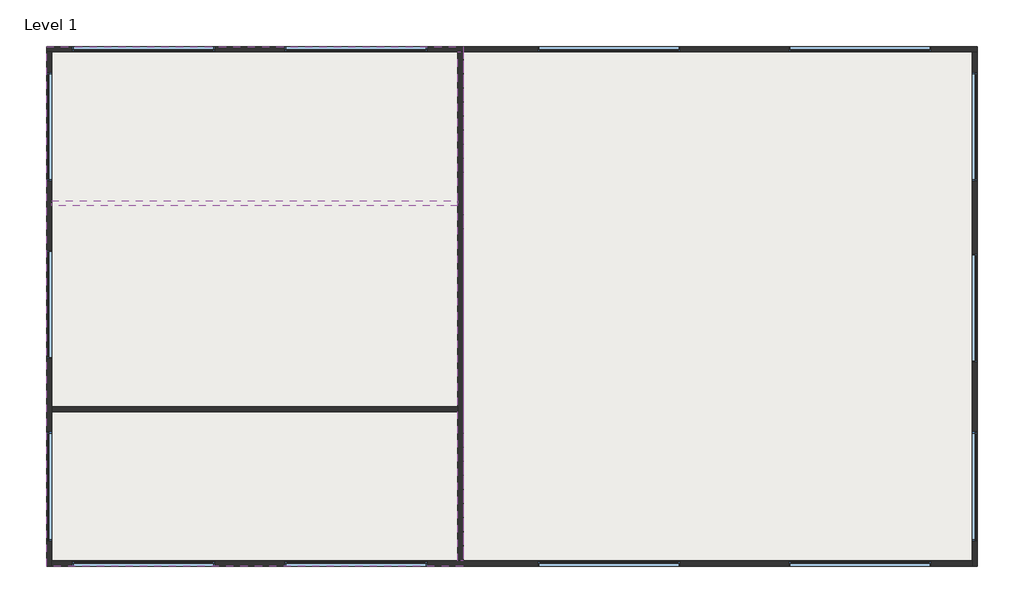
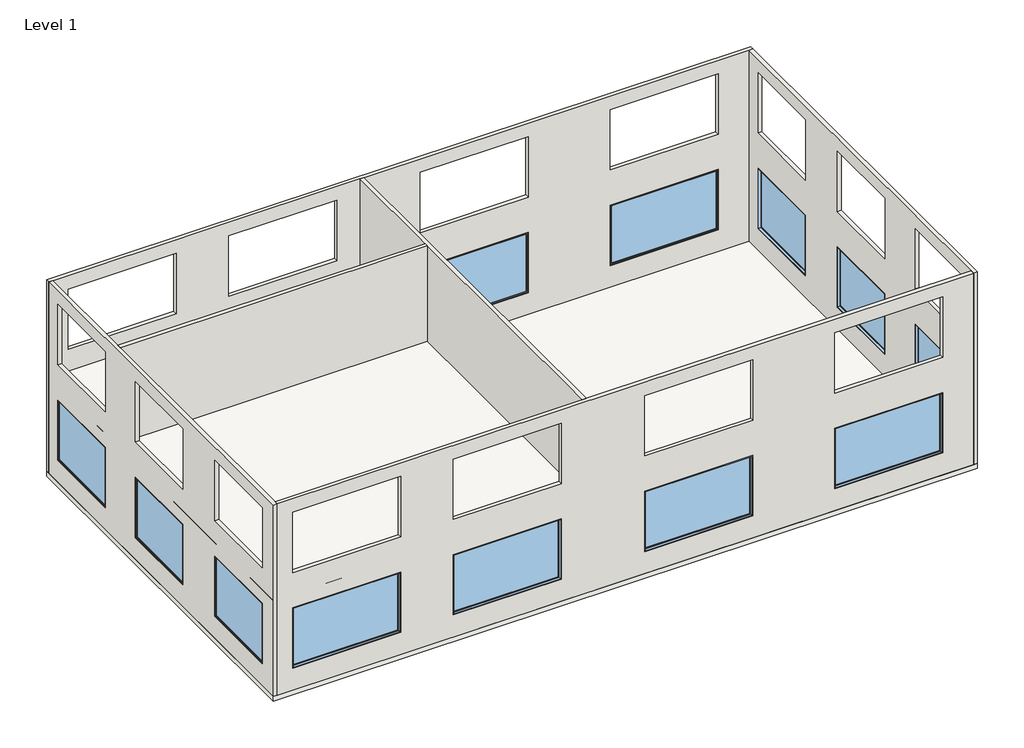
# One storey: 14 windows, 8 walls, 2 slabs.
"""IFC4 building model written with IfcOpenShell, lengths in millimetres."""

import ifcopenshell
import ifcopenshell.guid

model = None  # the IFC model being written
_history = None  # IfcOwnerHistory: only IFC2X3 demands one
_inside = {}  # id of a spatial element -> (the spatial element, [elements in it])
_under = {}  # id of a project, library or spatial element -> (it, [spatial elements below it])
_declared = {}  # id of a project -> (the project, [libraries it declares])
_typed = {}  # id of a type object -> (the type object, [elements of that type])
_made_of = {}  # id of a material, layer set ... -> (it, [elements and type objects made of it])


def new_model(schema):
    """Start an empty IFC model of exactly this schema.

    Asked for "IFC4X3", IfcOpenShell would pick the latest addendum, in which some entities
    have other attributes; the version numbers below select the first issue.
    IFC2X3 requires an IfcOwnerHistory on every rooted entity: one is made here for all.
    """
    global model, _history
    if schema == "IFC4X3":
        model = ifcopenshell.file(schema_version=(4, 3, 0, 0))
    else:
        model = ifcopenshell.file(schema=schema)
    _inside.clear()
    _under.clear()
    _declared.clear()
    _typed.clear()
    _made_of.clear()
    _history = None
    if model.schema == "IFC2X3":
        org = make("IfcOrganization", Name="unknown")
        user = make(
            "IfcPersonAndOrganization",
            ThePerson=make("IfcPerson", FamilyName="unknown"),
            TheOrganization=org,
        )
        app = make(
            "IfcApplication",
            ApplicationDeveloper=org,
            Version="unknown",
            ApplicationFullName="unknown",
            ApplicationIdentifier="unknown",
        )
        _history = make(
            "IfcOwnerHistory",
            OwningUser=user,
            OwningApplication=app,
            ChangeAction="ADDED",
            CreationDate=0,
        )
    return model


def make(cls, **values):
    """One entity of the class cls with the attributes given. An attribute that is None is left unset."""
    return model.create_entity(
        cls, **{name: value for name, value in values.items() if value is not None}
    )


def rooted(cls, **values):
    """An entity with a GlobalId (a new one), such as an element, a storey or a relation."""
    return make(cls, GlobalId=ifcopenshell.guid.new(), OwnerHistory=_history, **values)


def si_unit(unit_type, name, prefix=None):
    """IfcSIUnit, for example si_unit("LENGTHUNIT", "METRE", prefix="MILLI")."""
    return make("IfcSIUnit", UnitType=unit_type, Prefix=prefix, Name=name)


def assignment(units):
    """IfcUnitAssignment: the units of a project."""
    return None if units is None else make("IfcUnitAssignment", Units=units)


def point(xyz):
    """IfcCartesianPoint."""
    return None if xyz is None else make("IfcCartesianPoint", Coordinates=xyz)


def direction(xyz):
    """IfcDirection."""
    return None if xyz is None else make("IfcDirection", DirectionRatios=xyz)


def frame(location, z_axis=None, x_axis=None):
    """IfcAxis2Placement3D, a coordinate frame: its origin and axes. An axis left out is left unset."""
    return make(
        "IfcAxis2Placement3D",
        Location=point(location),
        Axis=direction(z_axis),
        RefDirection=direction(x_axis),
    )


def origin():
    """The frame at (0, 0, 0) with its axes left unset."""
    return frame((0.0, 0.0, 0.0))


def origin_with_axes():
    """The frame at (0, 0, 0) with the z axis (0, 0, 1) and the x axis (1, 0, 0) written out."""
    return frame((0.0, 0.0, 0.0), z_axis=(0.0, 0.0, 1.0), x_axis=(1.0, 0.0, 0.0))


def place(relative_to, where):
    """IfcLocalPlacement: puts the frame where relative to a parent placement (None: the world)."""
    return make(
        "IfcLocalPlacement", PlacementRelTo=relative_to, RelativePlacement=where
    )


def context(
    kind, dimensions, precision=None, world=None, true_north=None, identifier=None
):
    """IfcGeometricRepresentationContext, for example the 3D "Model" context."""
    return make(
        "IfcGeometricRepresentationContext",
        ContextIdentifier=identifier,
        ContextType=kind,
        CoordinateSpaceDimension=dimensions,
        Precision=precision,
        WorldCoordinateSystem=world,
        TrueNorth=true_north,
    )


def project(units=None, contexts=None):
    """IfcProject with its units and contexts."""
    return rooted(
        "IfcProject",
        Name="project",
        RepresentationContexts=contexts,
        UnitsInContext=assignment(units),
    )


def spatial(cls, under=None, at=None, **own):
    """A site, building, storey or space (cls), placed at a placement, below another one or the project."""
    s = rooted(cls, ObjectPlacement=at, **own)
    if under is not None:
        _under.setdefault(under.id(), (under, []))[1].append(s)
    return s


def polyline(points):
    """IfcPolyline through the points."""
    return make("IfcPolyline", Points=[point(p) for p in points])


def outline(outer, holes=None, kind="AREA"):
    """IfcArbitraryClosedProfileDef: a profile drawn as a closed curve; with holes, ...WithVoids."""
    if holes is None:
        return make("IfcArbitraryClosedProfileDef", ProfileType=kind, OuterCurve=outer)
    return make(
        "IfcArbitraryProfileDefWithVoids",
        ProfileType=kind,
        OuterCurve=outer,
        InnerCurves=holes,
    )


def extrude(swept, where, along, depth):
    """IfcExtrudedAreaSolid: the profile swept, set in the frame where, extruded along a direction by depth."""
    return make(
        "IfcExtrudedAreaSolid",
        SweptArea=swept,
        Position=where,
        ExtrudedDirection=direction(along),
        Depth=depth,
    )


def faces_of(points, faces, orient=None, outer=None):
    """IfcFace entities. A face is a list of loops; a loop is a list of indices into points, from 0.

    orient and outer hold one flag for each loop. By default every Orientation is true, the
    first loop of a face is its IfcFaceOuterBound and the others are IfcFaceBound.
    """
    made = []
    for i, loops in enumerate(faces):
        bounds = []
        for j, loop in enumerate(loops):
            is_outer = j == 0 if outer is None else outer[i][j]
            bounds.append(
                make(
                    "IfcFaceOuterBound" if is_outer else "IfcFaceBound",
                    Bound=make("IfcPolyLoop", Polygon=[points[k] for k in loop]),
                    Orientation=True if orient is None else orient[i][j],
                )
            )
        made.append(make("IfcFace", Bounds=bounds))
    return made


def faceted_brep(points, faces, orient=None, outer=None, voids=None):
    """IfcFacetedBrep: a solid bounded by flat faces; with voids (closed shells), ...WithVoids."""
    shared = [point(p) for p in points]
    hull = make("IfcClosedShell", CfsFaces=faces_of(shared, faces, orient, outer))
    if voids is None:
        return make("IfcFacetedBrep", Outer=hull)
    return make(
        "IfcFacetedBrepWithVoids",
        Outer=hull,
        Voids=[
            make(cls, CfsFaces=faces_of(shared, fs, o, b)) for cls, fs, o, b in voids
        ],
    )


def shape(context_of_items, identifier, shape_type, items):
    """IfcShapeRepresentation: the items that make up one representation, for example the "Body"."""
    return make(
        "IfcShapeRepresentation",
        ContextOfItems=context_of_items,
        RepresentationIdentifier=identifier,
        RepresentationType=shape_type,
        Items=items,
    )


def source(mapping_origin, context_of_items, identifier, shape_type, items):
    """IfcRepresentationMap: a shape defined once, which mapped items show again and again."""
    return make(
        "IfcRepresentationMap",
        MappingOrigin=mapping_origin,
        MappedRepresentation=shape(context_of_items, identifier, shape_type, items),
    )


def transform(
    local_origin,
    x_axis=None,
    y_axis=None,
    z_axis=None,
    scale=None,
    scale2=None,
    scale3=None,
    uniform=True,
):
    """IfcCartesianTransformationOperator3D, or its non-uniform kind. x_axis, y_axis, z_axis: its Axis1, 2, 3."""
    if uniform:
        return make(
            "IfcCartesianTransformationOperator3D",
            Axis1=direction(x_axis),
            Axis2=direction(y_axis),
            LocalOrigin=point(local_origin),
            Scale=scale,
            Axis3=direction(z_axis),
        )
    return make(
        "IfcCartesianTransformationOperator3DnonUniform",
        Axis1=direction(x_axis),
        Axis2=direction(y_axis),
        LocalOrigin=point(local_origin),
        Scale=scale,
        Axis3=direction(z_axis),
        Scale2=scale2,
        Scale3=scale3,
    )


def mapped(mapping_source, mapping_target):
    """IfcMappedItem: shows the shape of a source again, moved by a transform."""
    return make(
        "IfcMappedItem", MappingSource=mapping_source, MappingTarget=mapping_target
    )


def made_of(thing, what):
    """Note that an element or type object is made of a material, layer set ...; save() writes the relation."""
    if what is not None:
        _made_of.setdefault(what.id(), (what, []))[1].append(thing)
    return thing


def element(
    cls,
    number,
    at=None,
    inside=None,
    cuts=None,
    type_object=None,
    material=None,
    context=None,
    identifier="Body",
    shape_type=None,
    held_by="IfcProductDefinitionShape",
    body=None,
    shapes=None,
    **own,
):
    """One element of the class cls, such as IfcWall. Its Tag is "e" and its number.

    at: its placement. inside: the storey or other place that contains it. cuts: it is an
    opening in that element (IfcRelVoidsElement). A single representation is given by context,
    identifier, shape_type and body (its items); several are given by shapes. held_by: the class
    of the entity that holds the representations. save() writes the other relations.
    """
    e = rooted(cls, Tag="e%d" % number, ObjectPlacement=at, **own)
    if body is not None:
        shapes = [shape(context, identifier, shape_type, body)]
    if shapes is not None:
        e.Representation = make(held_by, Representations=shapes)
    if inside is not None:
        _inside.setdefault(inside.id(), (inside, []))[1].append(e)
    if cuts is not None:
        rooted(
            "IfcRelVoidsElement", RelatingBuildingElement=cuts, RelatedOpeningElement=e
        )
    if type_object is not None:
        _typed.setdefault(type_object.id(), (type_object, []))[1].append(e)
    return made_of(e, material)


def aggregate(whole, parts):
    """IfcRelAggregates: a whole, such as a stair, and the parts it consists of."""
    return rooted("IfcRelAggregates", RelatingObject=whole, RelatedObjects=parts)


def save(model, path):
    """Write the relations noted so far, then the file.

    IfcRelAggregates (storeys below a building ...), IfcRelContainedInSpatialStructure (elements
    in a storey), IfcRelDefinesByType, IfcRelAssociatesMaterial and IfcRelDeclares: one each for
    every whole, place, type object, material and project.
    """
    for whole, parts in _under.values():
        aggregate(whole, parts)
    for where, things in _inside.values():
        rooted(
            "IfcRelContainedInSpatialStructure",
            RelatedElements=things,
            RelatingStructure=where,
        )
    for kind, things in _typed.values():
        rooted("IfcRelDefinesByType", RelatedObjects=things, RelatingType=kind)
    for what, things in _made_of.values():
        rooted("IfcRelAssociatesMaterial", RelatedObjects=things, RelatingMaterial=what)
    for by, libraries in _declared.values():
        rooted("IfcRelDeclares", RelatingContext=by, RelatedDefinitions=libraries)
    model.write(path)


def m_fixed_2500x_4228mm_fd5e51e7(model_context):
    return source(origin(), model_context, "Body", "SweptSolid", [
        extrude(outline(polyline([(-2050.8, 54.2), (2050.8, 54.2), (2050.8, 42.2), (-2050.8, 42.2), (-2050.8, 54.2)])), frame((0.0, 0.0, 368.0), z_axis=(0.0, 0.0, 1.0), x_axis=(1.0, 0.0, 0.0)), (0.0, 0.0, 1.0), 2374.0),
        extrude(outline(polyline([(2786.0, -2094.8), (324.0, -2094.8), (324.0, 2094.8), (2786.0, 2094.8), (2786.0, -2094.8)]), holes=[polyline([(2742.0, -2050.8), (2742.0, 2050.8), (368.0, 2050.8), (368.0, -2050.8), (2742.0, -2050.8)])]), frame((0.0, 26.2, 0.0), z_axis=(0.0, 1.0, 0.0), x_axis=(0.0, 0.0, 1.0)), (0.0, 0.0, 1.0), 44.0),
        extrude(outline(polyline([(2805.0, -2113.8), (305.0, -2113.8), (305.0, 2113.8), (2805.0, 2113.8), (2805.0, -2113.8)]), holes=[polyline([(2786.0, -2094.8), (2786.0, 2094.8), (324.0, 2094.8), (324.0, -2094.8), (2786.0, -2094.8)])]), frame((0.0, 26.2, 0.0), z_axis=(0.0, 1.0, 0.0), x_axis=(0.0, 0.0, 1.0)), (0.0, 0.0, 1.0), 63.0),
        extrude(outline(polyline([(2805.0, -2113.8), (305.0, -2113.8), (305.0, 2113.8), (2805.0, 2113.8), (2805.0, -2113.8)]), holes=[polyline([(2773.0, -2081.8), (2773.0, 2081.8), (337.0, 2081.8), (337.0, -2081.8), (2773.0, -2081.8)])]), frame((0.0, -63.2, 0.0), z_axis=(0.0, 1.0, 0.0), x_axis=(0.0, 0.0, 1.0)), (0.0, 0.0, 1.0), 89.4),
    ])


def m_fixed_2500x_4228mm_f14c179f(model_context):
    return source(origin(), model_context, "Body", "SweptSolid", [
        extrude(outline(polyline([(-2050.8, -54.2), (-2050.8, -42.2), (2050.8, -42.2), (2050.8, -54.2), (-2050.8, -54.2)])), frame((0.0, 0.0, 368.0), z_axis=(0.0, 0.0, 1.0), x_axis=(1.0, 0.0, 0.0)), (0.0, 0.0, 1.0), 2374.0),
        extrude(outline(polyline([(2786.0, -2094.8), (324.0, -2094.8), (324.0, 2094.8), (2786.0, 2094.8), (2786.0, -2094.8)]), holes=[polyline([(2742.0, -2050.8), (2742.0, 2050.8), (368.0, 2050.8), (368.0, -2050.8), (2742.0, -2050.8)])]), frame((0.0, -70.2, 0.0), z_axis=(0.0, 1.0, 0.0), x_axis=(0.0, 0.0, 1.0)), (0.0, 0.0, 1.0), 44.0),
        extrude(outline(polyline([(2805.0, -2113.8), (305.0, -2113.8), (305.0, 2113.8), (2805.0, 2113.8), (2805.0, -2113.8)]), holes=[polyline([(2786.0, -2094.8), (2786.0, 2094.8), (324.0, 2094.8), (324.0, -2094.8), (2786.0, -2094.8)])]), frame((0.0, -89.2, 0.0), z_axis=(0.0, 1.0, 0.0), x_axis=(0.0, 0.0, 1.0)), (0.0, 0.0, 1.0), 63.0),
        extrude(outline(polyline([(2805.0, -2113.8), (305.0, -2113.8), (305.0, 2113.8), (2805.0, 2113.8), (2805.0, -2113.8)]), holes=[polyline([(2773.0, -2081.8), (2773.0, 2081.8), (337.0, 2081.8), (337.0, -2081.8), (2773.0, -2081.8)])]), frame((0.0, -26.2, 0.0), z_axis=(0.0, 1.0, 0.0), x_axis=(0.0, 0.0, 1.0)), (0.0, 0.0, 1.0), 89.4),
    ])


def m_fixed_2500x_3220mm_df94f4d0(model_context):
    return source(origin(), model_context, "Body", "SweptSolid", [
        extrude(outline(polyline([(-1546.8, 54.2), (1546.8, 54.2), (1546.8, 42.2), (-1546.8, 42.2), (-1546.8, 54.2)])), frame((0.0, 0.0, 368.0), z_axis=(0.0, 0.0, 1.0), x_axis=(1.0, 0.0, 0.0)), (0.0, 0.0, 1.0), 2374.0),
        extrude(outline(polyline([(2786.0, -1590.8), (324.0, -1590.8), (324.0, 1590.8), (2786.0, 1590.8), (2786.0, -1590.8)]), holes=[polyline([(2742.0, -1546.8), (2742.0, 1546.8), (368.0, 1546.8), (368.0, -1546.8), (2742.0, -1546.8)])]), frame((0.0, 26.2, 0.0), z_axis=(0.0, 1.0, 0.0), x_axis=(0.0, 0.0, 1.0)), (0.0, 0.0, 1.0), 44.0),
        extrude(outline(polyline([(2805.0, -1609.8), (305.0, -1609.8), (305.0, 1609.8), (2805.0, 1609.8), (2805.0, -1609.8)]), holes=[polyline([(2786.0, -1590.8), (2786.0, 1590.8), (324.0, 1590.8), (324.0, -1590.8), (2786.0, -1590.8)])]), frame((0.0, 26.2, 0.0), z_axis=(0.0, 1.0, 0.0), x_axis=(0.0, 0.0, 1.0)), (0.0, 0.0, 1.0), 63.0),
        extrude(outline(polyline([(2805.0, -1609.8), (305.0, -1609.8), (305.0, 1609.8), (2805.0, 1609.8), (2805.0, -1609.8)]), holes=[polyline([(2773.0, -1577.8), (2773.0, 1577.8), (337.0, 1577.8), (337.0, -1577.8), (2773.0, -1577.8)])]), frame((0.0, -63.2, 0.0), z_axis=(0.0, 1.0, 0.0), x_axis=(0.0, 0.0, 1.0)), (0.0, 0.0, 1.0), 89.4),
    ])


def m_fixed_2500x_3220mm_8b997f8c(model_context):
    return source(origin(), model_context, "Body", "SweptSolid", [
        extrude(outline(polyline([(-1546.8, -54.2), (-1546.8, -42.2), (1546.8, -42.2), (1546.8, -54.2), (-1546.8, -54.2)])), frame((0.0, 0.0, 368.0), z_axis=(0.0, 0.0, 1.0), x_axis=(1.0, 0.0, 0.0)), (0.0, 0.0, 1.0), 2374.0),
        extrude(outline(polyline([(2786.0, -1590.8), (324.0, -1590.8), (324.0, 1590.8), (2786.0, 1590.8), (2786.0, -1590.8)]), holes=[polyline([(2742.0, -1546.8), (2742.0, 1546.8), (368.0, 1546.8), (368.0, -1546.8), (2742.0, -1546.8)])]), frame((0.0, -70.2, 0.0), z_axis=(0.0, 1.0, 0.0), x_axis=(0.0, 0.0, 1.0)), (0.0, 0.0, 1.0), 44.0),
        extrude(outline(polyline([(2805.0, -1609.8), (305.0, -1609.8), (305.0, 1609.8), (2805.0, 1609.8), (2805.0, -1609.8)]), holes=[polyline([(2786.0, -1590.8), (2786.0, 1590.8), (324.0, 1590.8), (324.0, -1590.8), (2786.0, -1590.8)])]), frame((0.0, -89.2, 0.0), z_axis=(0.0, 1.0, 0.0), x_axis=(0.0, 0.0, 1.0)), (0.0, 0.0, 1.0), 63.0),
        extrude(outline(polyline([(2805.0, -1609.8), (305.0, -1609.8), (305.0, 1609.8), (2805.0, 1609.8), (2805.0, -1609.8)]), holes=[polyline([(2773.0, -1577.8), (2773.0, 1577.8), (337.0, 1577.8), (337.0, -1577.8), (2773.0, -1577.8)])]), frame((0.0, -26.2, 0.0), z_axis=(0.0, 1.0, 0.0), x_axis=(0.0, 0.0, 1.0)), (0.0, 0.0, 1.0), 89.4),
    ])


model = new_model("IFC4")

# Units and contexts
model_context = context("Model", 3, world=origin())
ifc_project = project(units=[si_unit("LENGTHUNIT", "METRE", prefix="MILLI")], contexts=[model_context])

# Site, building, storey
site = spatial("IfcSite", under=ifc_project)
building = spatial("IfcBuilding", under=site)
storey = spatial("IfcBuildingStorey", under=building, Name="Level 1", Elevation=0.0)

# Slabs
placement = place(None, origin())
element("IfcSlab", 1, ObjectType="160mm Concrete With 50mm Metal Deck", at=placement, inside=storey, context=model_context, shape_type="Brep", body=[
    faceted_brep([(29068.464681, 11296.9802217, -210.0), (29068.464681, -4095.4197783, -210.0), (1484.064681, -4095.4197783, -210.0), (1484.064681, 11296.9802217, -210.0), (29068.464681, 11296.9802217, 0.0), (1484.064681, 11296.9802217, 0.0), (1484.064681, 11144.5802217, 0.0), (1484.064681, -4095.4197783, 0.0), (28916.064681, -4095.4197783, 0.0), (29068.464681, -4095.4197783, 0.0), (29068.464681, 11144.5802217, 0.0)], [[[0, 1, 2, 3]], [[4, 5, 6, 7, 8, 9, 10]], [[1, 0, 4, 10, 9]], [[2, 1, 9, 8, 7]], [[3, 2, 7, 6, 5]], [[0, 3, 5, 4]]]),
])
element("IfcSlab", 2, ObjectType="160mm Concrete With 50mm Metal Deck", at=placement, inside=storey, context=model_context, shape_type="SweptSolid", body=[
    extrude(outline(polyline([(13828.464681, 11296.9802217), (13828.464681, -4095.4197783), (1484.064681, -4095.4197783), (1484.064681, 11296.9802217), (13828.464681, 11296.9802217)])), frame((0.0, 0.0, 3752.4), z_axis=(0.0, 0.0, 1.0), x_axis=(1.0, 0.0, 0.0)), (0.0, 0.0, 1.0), 210.0),
])

# Walls
element("IfcWall", 3, ObjectType="Generic - 152.4mm", at=placement, inside=storey, context=model_context, shape_type="Brep", body=[
    faceted_brep([(1484.064681, 11144.5802217, 0.0), (1636.464681, 11144.5802217, 0.0), (13676.064681, 11144.5802217, 0.0), (13828.464681, 11144.5802217, 0.0), (28916.064681, 11144.5802217, 0.0), (29068.464681, 11144.5802217, 0.0), (29068.464681, 11144.5802217, 7924.8), (28916.064681, 11144.5802217, 7924.8), (13828.464681, 11144.5802217, 7924.8), (13676.064681, 11144.5802217, 7924.8), (1636.464681, 11144.5802217, 7924.8), (1484.064681, 11144.5802217, 7924.8), (6474.064681, 11144.5802217, 902.4), (2246.464681, 11144.5802217, 902.4), (2246.464681, 11144.5802217, 3402.4), (6474.064681, 11144.5802217, 3402.4), (12766.064681, 11144.5802217, 902.4), (8538.464681, 11144.5802217, 902.4), (8538.464681, 11144.5802217, 3402.4), (12766.064681, 11144.5802217, 3402.4), (20266.064681, 11144.5802217, 902.4), (16038.464681, 11144.5802217, 902.4), (16038.464681, 11144.5802217, 3402.4), (20266.064681, 11144.5802217, 3402.4), (27706.064681, 11144.5802217, 902.4), (23478.464681, 11144.5802217, 902.4), (23478.464681, 11144.5802217, 3402.4), (27706.064681, 11144.5802217, 3402.4), (27706.064681, 11144.5802217, 4862.4), (23478.464681, 11144.5802217, 4862.4), (23478.464681, 11144.5802217, 7362.4), (27706.064681, 11144.5802217, 7362.4), (20266.064681, 11144.5802217, 4862.4), (16038.464681, 11144.5802217, 4862.4), (16038.464681, 11144.5802217, 7362.4), (20266.064681, 11144.5802217, 7362.4), (12766.064681, 11144.5802217, 4862.4), (8538.464681, 11144.5802217, 4862.4), (8538.464681, 11144.5802217, 7362.4), (12766.064681, 11144.5802217, 7362.4), (6474.064681, 11144.5802217, 4862.4), (2246.464681, 11144.5802217, 4862.4), (2246.464681, 11144.5802217, 7362.4), (6474.064681, 11144.5802217, 7362.4), (1484.064681, 11296.9802217, 0.0), (1484.064681, 11296.9802217, 7924.8), (29068.464681, 11296.9802217, 7924.8), (29068.464681, 11296.9802217, 0.0), (6474.064681, 11296.9802217, 902.4), (6474.064681, 11296.9802217, 3402.4), (2246.464681, 11296.9802217, 3402.4), (2246.464681, 11296.9802217, 902.4), (12766.064681, 11296.9802217, 902.4), (12766.064681, 11296.9802217, 3402.4), (8538.464681, 11296.9802217, 3402.4), (8538.464681, 11296.9802217, 902.4), (20266.064681, 11296.9802217, 902.4), (20266.064681, 11296.9802217, 3402.4), (16038.464681, 11296.9802217, 3402.4), (16038.464681, 11296.9802217, 902.4), (27706.064681, 11296.9802217, 902.4), (27706.064681, 11296.9802217, 3402.4), (23478.464681, 11296.9802217, 3402.4), (23478.464681, 11296.9802217, 902.4), (27706.064681, 11296.9802217, 4862.4), (27706.064681, 11296.9802217, 7362.4), (23478.464681, 11296.9802217, 7362.4), (23478.464681, 11296.9802217, 4862.4), (20266.064681, 11296.9802217, 4862.4), (20266.064681, 11296.9802217, 7362.4), (16038.464681, 11296.9802217, 7362.4), (16038.464681, 11296.9802217, 4862.4), (12766.064681, 11296.9802217, 4862.4), (12766.064681, 11296.9802217, 7362.4), (8538.464681, 11296.9802217, 7362.4), (8538.464681, 11296.9802217, 4862.4), (6474.064681, 11296.9802217, 4862.4), (6474.064681, 11296.9802217, 7362.4), (2246.464681, 11296.9802217, 7362.4), (2246.464681, 11296.9802217, 4862.4)], [[[0, 1, 2, 3, 4, 5, 6, 7, 8, 9, 10, 11], [12, 13, 14, 15], [16, 17, 18, 19], [20, 21, 22, 23], [24, 25, 26, 27], [28, 29, 30, 31], [32, 33, 34, 35], [36, 37, 38, 39], [40, 41, 42, 43]], [[44, 45, 46, 47], [48, 49, 50, 51], [52, 53, 54, 55], [56, 57, 58, 59], [60, 61, 62, 63], [64, 65, 66, 67], [68, 69, 70, 71], [72, 73, 74, 75], [76, 77, 78, 79]], [[5, 4, 3, 2, 1, 0, 44, 47]], [[11, 10, 9, 8, 7, 6, 46, 45]], [[6, 5, 47, 46]], [[0, 11, 45, 44]], [[49, 48, 12, 15]], [[50, 49, 15, 14]], [[51, 50, 14, 13]], [[48, 51, 13, 12]], [[53, 52, 16, 19]], [[54, 53, 19, 18]], [[55, 54, 18, 17]], [[52, 55, 17, 16]], [[57, 56, 20, 23]], [[58, 57, 23, 22]], [[59, 58, 22, 21]], [[56, 59, 21, 20]], [[61, 60, 24, 27]], [[62, 61, 27, 26]], [[63, 62, 26, 25]], [[60, 63, 25, 24]], [[65, 64, 28, 31]], [[66, 65, 31, 30]], [[67, 66, 30, 29]], [[64, 67, 29, 28]], [[69, 68, 32, 35]], [[70, 69, 35, 34]], [[71, 70, 34, 33]], [[68, 71, 33, 32]], [[73, 72, 36, 39]], [[74, 73, 39, 38]], [[75, 74, 38, 37]], [[72, 75, 37, 36]], [[77, 76, 40, 43]], [[78, 77, 43, 42]], [[79, 78, 42, 41]], [[76, 79, 41, 40]]]),
])
element("IfcWall", 4, ObjectType="Generic - 152.4mm", at=placement, inside=storey, context=model_context, shape_type="Brep", body=[
    faceted_brep([(28916.064681, 11144.5802217, 0.0), (28916.064681, -3943.0197783, 0.0), (28916.064681, -4095.4197783, 0.0), (28916.064681, -4095.4197783, 7924.8), (28916.064681, -3943.0197783, 7924.8), (28916.064681, 11144.5802217, 7924.8), (28916.064681, -3343.0197783, 902.4), (28916.064681, -123.4197783, 902.4), (28916.064681, -123.4197783, 3402.4), (28916.064681, -3343.0197783, 3402.4), (28916.064681, 1942.9802217, 902.4), (28916.064681, 5162.5802217, 902.4), (28916.064681, 5162.5802217, 3402.4), (28916.064681, 1942.9802217, 3402.4), (28916.064681, 7310.9802217, 902.4), (28916.064681, 10530.5802217, 902.4), (28916.064681, 10530.5802217, 3402.4), (28916.064681, 7310.9802217, 3402.4), (28916.064681, -3343.0197783, 4864.8), (28916.064681, -123.4197783, 4864.8), (28916.064681, -123.4197783, 7364.8), (28916.064681, -3343.0197783, 7364.8), (28916.064681, 1942.9802217, 4864.8), (28916.064681, 5162.5802217, 4864.8), (28916.064681, 5162.5802217, 7364.8), (28916.064681, 1942.9802217, 7364.8), (28916.064681, 7310.9802217, 4864.8), (28916.064681, 10530.5802217, 4864.8), (28916.064681, 10530.5802217, 7364.8), (28916.064681, 7310.9802217, 7364.8), (29068.464681, 11144.5802217, 0.0), (29068.464681, 11144.5802217, 7924.8), (29068.464681, -4095.4197783, 7924.8), (29068.464681, -4095.4197783, 0.0), (29068.464681, -3343.0197783, 902.4), (29068.464681, -3343.0197783, 3402.4), (29068.464681, -123.4197783, 3402.4), (29068.464681, -123.4197783, 902.4), (29068.464681, 1942.9802217, 902.4), (29068.464681, 1942.9802217, 3402.4), (29068.464681, 5162.5802217, 3402.4), (29068.464681, 5162.5802217, 902.4), (29068.464681, 7310.9802217, 902.4), (29068.464681, 7310.9802217, 3402.4), (29068.464681, 10530.5802217, 3402.4), (29068.464681, 10530.5802217, 902.4), (29068.464681, -3343.0197783, 4864.8), (29068.464681, -3343.0197783, 7364.8), (29068.464681, -123.4197783, 7364.8), (29068.464681, -123.4197783, 4864.8), (29068.464681, 1942.9802217, 4864.8), (29068.464681, 1942.9802217, 7364.8), (29068.464681, 5162.5802217, 7364.8), (29068.464681, 5162.5802217, 4864.8), (29068.464681, 7310.9802217, 4864.8), (29068.464681, 7310.9802217, 7364.8), (29068.464681, 10530.5802217, 7364.8), (29068.464681, 10530.5802217, 4864.8)], [[[0, 1, 2, 3, 4, 5], [6, 7, 8, 9], [10, 11, 12, 13], [14, 15, 16, 17], [18, 19, 20, 21], [22, 23, 24, 25], [26, 27, 28, 29]], [[30, 31, 32, 33], [34, 35, 36, 37], [38, 39, 40, 41], [42, 43, 44, 45], [46, 47, 48, 49], [50, 51, 52, 53], [54, 55, 56, 57]], [[2, 1, 0, 30, 33]], [[5, 4, 3, 32, 31]], [[0, 5, 31, 30]], [[35, 34, 6, 9]], [[36, 35, 9, 8]], [[37, 36, 8, 7]], [[34, 37, 7, 6]], [[39, 38, 10, 13]], [[40, 39, 13, 12]], [[41, 40, 12, 11]], [[38, 41, 11, 10]], [[43, 42, 14, 17]], [[44, 43, 17, 16]], [[45, 44, 16, 15]], [[42, 45, 15, 14]], [[3, 2, 33, 32]], [[47, 46, 18, 21]], [[48, 47, 21, 20]], [[49, 48, 20, 19]], [[46, 49, 19, 18]], [[51, 50, 22, 25]], [[52, 51, 25, 24]], [[53, 52, 24, 23]], [[50, 53, 23, 22]], [[55, 54, 26, 29]], [[56, 55, 29, 28]], [[57, 56, 28, 27]], [[54, 57, 27, 26]]]),
])
element("IfcWall", 5, ObjectType="Generic - 152.4mm", at=placement, inside=storey, context=model_context, shape_type="Brep", body=[
    faceted_brep([(28916.064681, -3943.0197783, 0.0), (13828.464681, -3943.0197783, 0.0), (13676.064681, -3943.0197783, 0.0), (1636.464681, -3943.0197783, 0.0), (1636.464681, -3943.0197783, 7924.8), (13676.064681, -3943.0197783, 7924.8), (13828.464681, -3943.0197783, 7924.8), (28916.064681, -3943.0197783, 7924.8), (27706.064681, -3943.0197783, 902.4), (27706.064681, -3943.0197783, 3402.4), (23478.464681, -3943.0197783, 3402.4), (23478.464681, -3943.0197783, 902.4), (20266.064681, -3943.0197783, 902.4), (20266.064681, -3943.0197783, 3402.4), (16038.464681, -3943.0197783, 3402.4), (16038.464681, -3943.0197783, 902.4), (12766.064681, -3943.0197783, 902.4), (12766.064681, -3943.0197783, 3402.4), (8538.464681, -3943.0197783, 3402.4), (8538.464681, -3943.0197783, 902.4), (6474.064681, -3943.0197783, 902.4), (6474.064681, -3943.0197783, 3402.4), (2246.464681, -3943.0197783, 3402.4), (2246.464681, -3943.0197783, 902.4), (27706.064681, -3943.0197783, 4862.4), (27706.064681, -3943.0197783, 7362.4), (23478.464681, -3943.0197783, 7362.4), (23478.464681, -3943.0197783, 4862.4), (20266.064681, -3943.0197783, 4862.4), (20266.064681, -3943.0197783, 7362.4), (16038.464681, -3943.0197783, 7362.4), (16038.464681, -3943.0197783, 4862.4), (12766.064681, -3943.0197783, 4862.4), (12766.064681, -3943.0197783, 7362.4), (8538.464681, -3943.0197783, 7362.4), (8538.464681, -3943.0197783, 4862.4), (6474.064681, -3943.0197783, 4862.4), (6474.064681, -3943.0197783, 7362.4), (2246.464681, -3943.0197783, 7362.4), (2246.464681, -3943.0197783, 4862.4), (28916.064681, -4095.4197783, 0.0), (28916.064681, -4095.4197783, 7924.8), (1636.464681, -4095.4197783, 7924.8), (1636.464681, -4095.4197783, 0.0), (27706.064681, -4095.4197783, 902.4), (23478.464681, -4095.4197783, 902.4), (23478.464681, -4095.4197783, 3402.4), (27706.064681, -4095.4197783, 3402.4), (20266.064681, -4095.4197783, 902.4), (16038.464681, -4095.4197783, 902.4), (16038.464681, -4095.4197783, 3402.4), (20266.064681, -4095.4197783, 3402.4), (12766.064681, -4095.4197783, 902.4), (8538.464681, -4095.4197783, 902.4), (8538.464681, -4095.4197783, 3402.4), (12766.064681, -4095.4197783, 3402.4), (6474.064681, -4095.4197783, 902.4), (2246.464681, -4095.4197783, 902.4), (2246.464681, -4095.4197783, 3402.4), (6474.064681, -4095.4197783, 3402.4), (27706.064681, -4095.4197783, 4862.4), (23478.464681, -4095.4197783, 4862.4), (23478.464681, -4095.4197783, 7362.4), (27706.064681, -4095.4197783, 7362.4), (20266.064681, -4095.4197783, 4862.4), (16038.464681, -4095.4197783, 4862.4), (16038.464681, -4095.4197783, 7362.4), (20266.064681, -4095.4197783, 7362.4), (12766.064681, -4095.4197783, 4862.4), (8538.464681, -4095.4197783, 4862.4), (8538.464681, -4095.4197783, 7362.4), (12766.064681, -4095.4197783, 7362.4), (6474.064681, -4095.4197783, 4862.4), (2246.464681, -4095.4197783, 4862.4), (2246.464681, -4095.4197783, 7362.4), (6474.064681, -4095.4197783, 7362.4)], [[[0, 1, 2, 3, 4, 5, 6, 7], [8, 9, 10, 11], [12, 13, 14, 15], [16, 17, 18, 19], [20, 21, 22, 23], [24, 25, 26, 27], [28, 29, 30, 31], [32, 33, 34, 35], [36, 37, 38, 39]], [[40, 41, 42, 43], [44, 45, 46, 47], [48, 49, 50, 51], [52, 53, 54, 55], [56, 57, 58, 59], [60, 61, 62, 63], [64, 65, 66, 67], [68, 69, 70, 71], [72, 73, 74, 75]], [[3, 2, 1, 0, 40, 43]], [[7, 6, 5, 4, 42, 41]], [[9, 8, 44, 47]], [[10, 9, 47, 46]], [[11, 10, 46, 45]], [[8, 11, 45, 44]], [[13, 12, 48, 51]], [[14, 13, 51, 50]], [[15, 14, 50, 49]], [[12, 15, 49, 48]], [[17, 16, 52, 55]], [[18, 17, 55, 54]], [[19, 18, 54, 53]], [[16, 19, 53, 52]], [[21, 20, 56, 59]], [[22, 21, 59, 58]], [[23, 22, 58, 57]], [[20, 23, 57, 56]], [[0, 7, 41, 40]], [[4, 3, 43, 42]], [[25, 24, 60, 63]], [[26, 25, 63, 62]], [[27, 26, 62, 61]], [[24, 27, 61, 60]], [[29, 28, 64, 67]], [[30, 29, 67, 66]], [[31, 30, 66, 65]], [[28, 31, 65, 64]], [[33, 32, 68, 71]], [[34, 33, 71, 70]], [[35, 34, 70, 69]], [[32, 35, 69, 68]], [[37, 36, 72, 75]], [[38, 37, 75, 74]], [[39, 38, 74, 73]], [[36, 39, 73, 72]]]),
])
element("IfcWall", 6, ObjectType="Generic - 152.4mm", at=placement, inside=storey, context=model_context, shape_type="Brep", body=[
    faceted_brep([(1636.464681, -4095.4197783, 0.0), (1636.464681, -3943.0197783, 0.0), (1636.464681, 476.5802217, 0.0), (1636.464681, 628.9802217, 0.0), (1636.464681, 11144.5802217, 0.0), (1636.464681, 11144.5802217, 7924.8), (1636.464681, 6724.9802217, 7924.8), (1636.464681, 6572.5802217, 7924.8), (1636.464681, -3943.0197783, 7924.8), (1636.464681, -4095.4197783, 7924.8), (1636.464681, 7310.9802217, 902.4), (1636.464681, 7310.9802217, 3402.4), (1636.464681, 10530.5802217, 3402.4), (1636.464681, 10530.5802217, 902.4), (1636.464681, 2042.9802217, 902.4), (1636.464681, 2042.9802217, 3402.4), (1636.464681, 5262.5802217, 3402.4), (1636.464681, 5262.5802217, 902.4), (1636.464681, -3343.0197783, 902.4), (1636.464681, -3343.0197783, 3402.4), (1636.464681, -123.4197783, 3402.4), (1636.464681, -123.4197783, 902.4), (1636.464681, -3343.0197783, 4864.8), (1636.464681, -3343.0197783, 7364.8), (1636.464681, -123.4197783, 7364.8), (1636.464681, -123.4197783, 4864.8), (1636.464681, 2042.9802217, 4864.8), (1636.464681, 2042.9802217, 7364.8), (1636.464681, 5262.5802217, 7364.8), (1636.464681, 5262.5802217, 4864.8), (1636.464681, 7310.9802217, 4864.8), (1636.464681, 7310.9802217, 7364.8), (1636.464681, 10530.5802217, 7364.8), (1636.464681, 10530.5802217, 4864.8), (1484.064681, -4095.4197783, 0.0), (1484.064681, -4095.4197783, 7924.8), (1484.064681, 11144.5802217, 7924.8), (1484.064681, 11144.5802217, 0.0), (1484.064681, 7310.9802217, 902.4), (1484.064681, 10530.5802217, 902.4), (1484.064681, 10530.5802217, 3402.4), (1484.064681, 7310.9802217, 3402.4), (1484.064681, 2042.9802217, 902.4), (1484.064681, 5262.5802217, 902.4), (1484.064681, 5262.5802217, 3402.4), (1484.064681, 2042.9802217, 3402.4), (1484.064681, -3343.0197783, 902.4), (1484.064681, -123.4197783, 902.4), (1484.064681, -123.4197783, 3402.4), (1484.064681, -3343.0197783, 3402.4), (1484.064681, -3343.0197783, 4864.8), (1484.064681, -123.4197783, 4864.8), (1484.064681, -123.4197783, 7364.8), (1484.064681, -3343.0197783, 7364.8), (1484.064681, 2042.9802217, 4864.8), (1484.064681, 5262.5802217, 4864.8), (1484.064681, 5262.5802217, 7364.8), (1484.064681, 2042.9802217, 7364.8), (1484.064681, 7310.9802217, 4864.8), (1484.064681, 10530.5802217, 4864.8), (1484.064681, 10530.5802217, 7364.8), (1484.064681, 7310.9802217, 7364.8)], [[[0, 1, 2, 3, 4, 5, 6, 7, 8, 9], [10, 11, 12, 13], [14, 15, 16, 17], [18, 19, 20, 21], [22, 23, 24, 25], [26, 27, 28, 29], [30, 31, 32, 33]], [[34, 35, 36, 37], [38, 39, 40, 41], [42, 43, 44, 45], [46, 47, 48, 49], [50, 51, 52, 53], [54, 55, 56, 57], [58, 59, 60, 61]], [[4, 3, 2, 1, 0, 34, 37]], [[9, 8, 7, 6, 5, 36, 35]], [[5, 4, 37, 36]], [[11, 10, 38, 41]], [[12, 11, 41, 40]], [[13, 12, 40, 39]], [[10, 13, 39, 38]], [[15, 14, 42, 45]], [[16, 15, 45, 44]], [[17, 16, 44, 43]], [[14, 17, 43, 42]], [[19, 18, 46, 49]], [[20, 19, 49, 48]], [[21, 20, 48, 47]], [[18, 21, 47, 46]], [[0, 9, 35, 34]], [[23, 22, 50, 53]], [[24, 23, 53, 52]], [[25, 24, 52, 51]], [[22, 25, 51, 50]], [[27, 26, 54, 57]], [[28, 27, 57, 56]], [[29, 28, 56, 55]], [[26, 29, 55, 54]], [[31, 30, 58, 61]], [[32, 31, 61, 60]], [[33, 32, 60, 59]], [[30, 33, 59, 58]]]),
])
element("IfcWall", 7, ObjectType="Generic - 152.4mm - Interior", at=placement, inside=storey, context=model_context, shape_type="Brep", body=[
    faceted_brep([(13828.464681, -3943.0197783, 0.0), (13828.464681, 11144.5802217, 0.0), (13828.464681, 11144.5802217, 3752.4), (13828.464681, -3943.0197783, 3752.4), (13676.064681, -3943.0197783, 0.0), (13676.064681, -3943.0197783, 3752.4), (13676.064681, 476.5802217, 3752.4), (13676.064681, 628.9802217, 3752.4), (13676.064681, 11144.5802217, 3752.4), (13676.064681, 11144.5802217, 0.0), (13676.064681, 628.9802217, 0.0), (13676.064681, 476.5802217, 0.0)], [[[0, 1, 2, 3]], [[4, 5, 6, 7, 8, 9, 10, 11]], [[1, 0, 4, 11, 10, 9]], [[0, 3, 5, 4]], [[2, 1, 9, 8]], [[3, 2, 8, 7, 6, 5]]]),
])
element("IfcWall", 8, ObjectType="Generic - 152.4mm - Interior", at=placement, inside=storey, context=model_context, shape_type="SweptSolid", body=[
    extrude(outline(polyline([(1636.464681, 628.9802217), (13676.064681, 628.9802217), (13676.064681, 476.5802217), (1636.464681, 476.5802217), (1636.464681, 628.9802217)])), origin_with_axes(), (0.0, 0.0, 1.0), 3752.4),
])
element("IfcWall", 9, ObjectType="Generic - 152.4mm - Interior", at=placement, inside=storey, context=model_context, shape_type="Brep", body=[
    faceted_brep([(13676.064681, 11144.5802217, 3962.4), (13676.064681, 6724.9802217, 3962.4), (13676.064681, 6572.5802217, 3962.4), (13676.064681, -3943.0197783, 3962.4), (13676.064681, -3943.0197783, 7924.8), (13676.064681, 6572.5802217, 7924.8), (13676.064681, 6724.9802217, 7924.8), (13676.064681, 11144.5802217, 7924.8), (13828.464681, 11144.5802217, 3962.4), (13828.464681, 11144.5802217, 7924.8), (13828.464681, -3943.0197783, 7924.8), (13828.464681, -3943.0197783, 3962.4)], [[[0, 1, 2, 3, 4, 5, 6, 7]], [[8, 9, 10, 11]], [[3, 2, 1, 0, 8, 11]], [[7, 6, 5, 4, 10, 9]], [[4, 3, 11, 10]], [[0, 7, 9, 8]]]),
])
element("IfcWall", 10, ObjectType="Generic - 152.4mm - Interior", at=placement, inside=storey, context=model_context, shape_type="SweptSolid", body=[
    extrude(outline(polyline([(1636.464681, 6724.9802217), (13676.064681, 6724.9802217), (13676.064681, 6572.5802217), (1636.464681, 6572.5802217), (1636.464681, 6724.9802217)])), frame((0.0, 0.0, 3962.4), z_axis=(0.0, 0.0, 1.0), x_axis=(1.0, 0.0, 0.0)), (0.0, 0.0, 1.0), 3962.4),
])

# Windows
m_fixed_2500x_4228mm_shape = m_fixed_2500x_4228mm_fd5e51e7(model_context)
element("IfcWindow", 11, ObjectType="M_Fixed : 2500X 4228mm", at=placement, inside=storey, context=model_context, shape_type="MappedRepresentation", body=[
    mapped(m_fixed_2500x_4228mm_shape, transform((4360.264681, 11233.7802217, 597.4), x_axis=(-1.0, 0.0, 0.0), y_axis=(0.0, -1.0, 0.0), z_axis=(0.0, 0.0, 1.0))),
])
element("IfcWindow", 12, ObjectType="M_Fixed : 2500X 4228mm", at=placement, inside=storey, context=model_context, shape_type="MappedRepresentation", body=[
    mapped(m_fixed_2500x_4228mm_shape, transform((10652.264681, 11233.7802217, 597.4), x_axis=(-1.0, 0.0, 0.0), y_axis=(0.0, -1.0, 0.0), z_axis=(0.0, 0.0, 1.0))),
])
element("IfcWindow", 13, ObjectType="M_Fixed : 2500X 4228mm", at=placement, inside=storey, context=model_context, shape_type="MappedRepresentation", body=[
    mapped(m_fixed_2500x_4228mm_shape, transform((18152.264681, 11233.7802217, 597.4), x_axis=(-1.0, 0.0, 0.0), y_axis=(0.0, -1.0, 0.0), z_axis=(0.0, 0.0, 1.0))),
])
element("IfcWindow", 14, ObjectType="M_Fixed : 2500X 4228mm", at=placement, inside=storey, context=model_context, shape_type="MappedRepresentation", body=[
    mapped(m_fixed_2500x_4228mm_shape, transform((25592.264681, 11233.7802217, 597.4), x_axis=(-1.0, 0.0, 0.0), y_axis=(0.0, -1.0, 0.0), z_axis=(0.0, 0.0, 1.0))),
])
m_fixed_2500x_4228mm_2_shape = m_fixed_2500x_4228mm_f14c179f(model_context)
element("IfcWindow", 15, ObjectType="M_Fixed : 2500X 4228mm", at=placement, inside=storey, context=model_context, shape_type="MappedRepresentation", body=[
    mapped(m_fixed_2500x_4228mm_2_shape, transform((4360.264681, -4032.2197783, 597.4), x_axis=(-1.0, 0.0, 0.0), y_axis=(0.0, -1.0, 0.0), z_axis=(0.0, 0.0, 1.0))),
])
element("IfcWindow", 16, ObjectType="M_Fixed : 2500X 4228mm", at=placement, inside=storey, context=model_context, shape_type="MappedRepresentation", body=[
    mapped(m_fixed_2500x_4228mm_2_shape, transform((10652.264681, -4032.2197783, 597.4), x_axis=(-1.0, 0.0, 0.0), y_axis=(0.0, -1.0, 0.0), z_axis=(0.0, 0.0, 1.0))),
])
element("IfcWindow", 17, ObjectType="M_Fixed : 2500X 4228mm", at=placement, inside=storey, context=model_context, shape_type="MappedRepresentation", body=[
    mapped(m_fixed_2500x_4228mm_2_shape, transform((18152.264681, -4032.2197783, 597.4), x_axis=(-1.0, 0.0, 0.0), y_axis=(0.0, -1.0, 0.0), z_axis=(0.0, 0.0, 1.0))),
])
element("IfcWindow", 18, ObjectType="M_Fixed : 2500X 4228mm", at=placement, inside=storey, context=model_context, shape_type="MappedRepresentation", body=[
    mapped(m_fixed_2500x_4228mm_2_shape, transform((25592.264681, -4032.2197783, 597.4), x_axis=(-1.0, 0.0, 0.0), y_axis=(0.0, -1.0, 0.0), z_axis=(0.0, 0.0, 1.0))),
])
m_fixed_2500x_3220mm_shape = m_fixed_2500x_3220mm_df94f4d0(model_context)
element("IfcWindow", 19, ObjectType="M_Fixed : 2500x 3220mm", at=placement, inside=storey, context=model_context, shape_type="MappedRepresentation", body=[
    mapped(m_fixed_2500x_3220mm_shape, transform((1573.264681, 8920.7802217, 597.4), x_axis=(0.0, 1.0, 0.0), y_axis=(-1.0, 0.0, 0.0), z_axis=(0.0, 0.0, 1.0))),
])
element("IfcWindow", 20, ObjectType="M_Fixed : 2500x 3220mm", at=placement, inside=storey, context=model_context, shape_type="MappedRepresentation", body=[
    mapped(m_fixed_2500x_3220mm_shape, transform((1573.264681, 3652.7802217, 597.4), x_axis=(0.0, 1.0, 0.0), y_axis=(-1.0, 0.0, 0.0), z_axis=(0.0, 0.0, 1.0))),
])
element("IfcWindow", 21, ObjectType="M_Fixed : 2500x 3220mm", at=placement, inside=storey, context=model_context, shape_type="MappedRepresentation", body=[
    mapped(m_fixed_2500x_3220mm_shape, transform((1573.264681, -1733.2197783, 597.4), x_axis=(0.0, 1.0, 0.0), y_axis=(-1.0, 0.0, 0.0), z_axis=(0.0, 0.0, 1.0))),
])
m_fixed_2500x_3220mm_2_shape = m_fixed_2500x_3220mm_8b997f8c(model_context)
element("IfcWindow", 22, ObjectType="M_Fixed : 2500x 3220mm", at=placement, inside=storey, context=model_context, shape_type="MappedRepresentation", body=[
    mapped(m_fixed_2500x_3220mm_2_shape, transform((28979.264681, 8920.7802217, 597.4), x_axis=(0.0, 1.0, 0.0), y_axis=(-1.0, 0.0, 0.0), z_axis=(0.0, 0.0, 1.0))),
])
element("IfcWindow", 23, ObjectType="M_Fixed : 2500x 3220mm", at=placement, inside=storey, context=model_context, shape_type="MappedRepresentation", body=[
    mapped(m_fixed_2500x_3220mm_2_shape, transform((28979.264681, 3552.7802217, 597.4), x_axis=(0.0, 1.0, 0.0), y_axis=(-1.0, 0.0, 0.0), z_axis=(0.0, 0.0, 1.0))),
])
element("IfcWindow", 24, ObjectType="M_Fixed : 2500x 3220mm", at=placement, inside=storey, context=model_context, shape_type="MappedRepresentation", body=[
    mapped(m_fixed_2500x_3220mm_2_shape, transform((28979.264681, -1733.2197783, 597.4), x_axis=(0.0, 1.0, 0.0), y_axis=(-1.0, 0.0, 0.0), z_axis=(0.0, 0.0, 1.0))),
])

save(model, "model.ifc")

# Revit data of these elements
# Project information
#   Project Issue Date = "Issue Date"
#   Project Status = "Project Status"
#   Client Name = "Owner"
#   Project Address = "Enter address here"
#   Project Name = "Project Name"
#   Project Number = "Project Number"
# Type "160mm Concrete With 50mm Metal Deck"
#   Function = 0
#   Layers, outside or top first: 210 mm no material (function 1); 0 mm "Metal Deck" (function 200)
# Type "Generic - 152.4mm"
#   Layers, outside or top first: 152.4 mm no material (function 1)
# Type "Generic - 152.4mm - Interior"
#   Layers, outside or top first: 152.4 mm no material (function 1)
# Type "M_Fixed : 2500X 4228mm"
#   Type Mark = "25"
#   Height = 2500 mm
#   Default Sill Height = 305 mm
#   Width = 4227.6 mm
#   Window Inset = 19 mm
#   Frame Exterior Material = Sash
#   Frame Interior Material = Sash
#   Glass Pane Material = Glass
#   Sash = Sash
#   Wall Closure = (empty or 0)
# Type "M_Fixed : 2500x 3220mm"
#   Type Mark = "26"
#   Height = 2500 mm
#   Default Sill Height = 305 mm
#   Width = 3219.6 mm
#   Window Inset = 19 mm
#   Frame Exterior Material = Sash
#   Frame Interior Material = Sash
#   Glass Pane Material = Glass
#   Sash = Sash
#   Wall Closure = (empty or 0)
# Element 1 (IfcSlab, "160mm Concrete With 50mm Metal Deck")
#   Height Offset From Level = 0 mm
#   Phase Created = New Construction
#   Materials on its faces: "Metal Deck", "Default Floor"
# Element 2 (IfcSlab, "160mm Concrete With 50mm Metal Deck")
#   Height Offset From Level = 3962.4 mm
#   Phase Created = New Construction
#   Materials on its faces: "Metal Deck", "Default Floor"
# Elements 3, 4, 5, 6 (IfcWall, "Generic - 152.4mm")
#   Top Offset = 0 mm
#   Base Offset = 0 mm
#   wall height = 7924.8 mm
#   Phase Created = New Construction
#   Base Constraint = Level 1
#   Top Constraint = Roof Level
#   Materials on its faces: "Default Wall"
# Element 7 (IfcWall, "Generic - 152.4mm - Interior")
#   Top Offset = 3962.4 mm
#   Base Offset = 0 mm
#   wall height = 3752.4 mm
#   Phase Created = New Construction
#   Base Constraint = Level 1
#   Top Constraint = Level 1
#   Materials on its faces: "Default Wall"
# Element 8 (IfcWall, "Generic - 152.4mm - Interior")
#   Top Offset = 3862.4 mm
#   Base Offset = 0 mm
#   wall height = 3752.4 mm
#   Phase Created = New Construction
#   Base Constraint = Level 1
#   Top Constraint = Level 1
#   Materials on its faces: "Default Wall"
# Elements 9, 10 (IfcWall, "Generic - 152.4mm - Interior")
#   built-in parameter 1001111 = 3962.4 mm
#   Top Offset = 0 mm
#   Base Offset = 3962.4 mm
#   Unconnected Height = 3962.4 mm
#   wall height = 3962.4 mm
#   Phase Created = New Construction
#   Base Constraint = Level 1
#   Top Constraint = Roof Level
#   Materials on its faces: "Default Wall"
# Element 11 (IfcWindow, "M_Fixed : 2500X 4228mm")
#   Mark = "10"
#   Phase Created = New Construction
#   Materials on its faces: "Sash", "Glass"
# Element 12 (IfcWindow, "M_Fixed : 2500X 4228mm")
#   Mark = "11"
#   Phase Created = New Construction
#   Materials on its faces: "Sash", "Glass"
# Element 13 (IfcWindow, "M_Fixed : 2500X 4228mm")
#   Mark = "12"
#   Phase Created = New Construction
#   Materials on its faces: "Sash", "Glass"
# Element 14 (IfcWindow, "M_Fixed : 2500X 4228mm")
#   Mark = "13"
#   Phase Created = New Construction
#   Materials on its faces: "Sash", "Glass"
# Element 15 (IfcWindow, "M_Fixed : 2500X 4228mm")
#   Mark = "14"
#   Phase Created = New Construction
#   Materials on its faces: "Sash", "Glass"
# Element 16 (IfcWindow, "M_Fixed : 2500X 4228mm")
#   Mark = "15"
#   Phase Created = New Construction
#   Materials on its faces: "Sash", "Glass"
# Element 17 (IfcWindow, "M_Fixed : 2500X 4228mm")
#   Mark = "16"
#   Phase Created = New Construction
#   Materials on its faces: "Sash", "Glass"
# Element 18 (IfcWindow, "M_Fixed : 2500X 4228mm")
#   Mark = "17"
#   Phase Created = New Construction
#   Materials on its faces: "Sash", "Glass"
# Element 19 (IfcWindow, "M_Fixed : 2500x 3220mm")
#   Mark = "27"
#   Phase Created = New Construction
#   Materials on its faces: "Sash", "Glass"
# Element 20 (IfcWindow, "M_Fixed : 2500x 3220mm")
#   Mark = "28"
#   Phase Created = New Construction
#   Materials on its faces: "Sash", "Glass"
# Element 21 (IfcWindow, "M_Fixed : 2500x 3220mm")
#   Mark = "29"
#   Phase Created = New Construction
#   Materials on its faces: "Sash", "Glass"
# Element 22 (IfcWindow, "M_Fixed : 2500x 3220mm")
#   Mark = "30"
#   Phase Created = New Construction
#   Materials on its faces: "Sash", "Glass"
# Element 23 (IfcWindow, "M_Fixed : 2500x 3220mm")
#   Mark = "31"
#   Phase Created = New Construction
#   Materials on its faces: "Sash", "Glass"
# Element 24 (IfcWindow, "M_Fixed : 2500x 3220mm")
#   Mark = "32"
#   Phase Created = New Construction
#   Materials on its faces: "Sash", "Glass"
# Materials
#   "Metal Deck": class "Metal", colour RGB 247 247 247, transparency 0, Description = "Steel, mill finish", Cost = 0
#   "Sash": class "Wood", colour RGB 136 99 55, transparency 0
#   "Glass": class "Glass", colour RGB 0 128 192, transparency 0.9, Description = "Soda Lime Glass", Cost = 0
#   "Default Floor": class "Miscellaneous", colour RGB 127 127 127, transparency 0, Cost = 0
#   "Default Wall": class "Miscellaneous", colour RGB 128 128 128, transparency 0, Cost = 0
# Room at (7259.725, -1600.456) mm, phase "New Construction", upper level "Level 2", upper offset 0 mm, lower offset 0 mm
#   Number = "6"
#   Name = "Room"
# Room at (8198.725, 4816.984) mm, phase "New Construction", upper level "Level 2", upper offset 0 mm, lower offset 0 mm
#   Number = "7"
#   Name = "Room"
# Room at (21274.823, 2677.837) mm, phase "New Construction", upper level "Roof Level", upper offset 0 mm, lower offset 0 mm
#   Number = "8"
#   Name = "Room"
